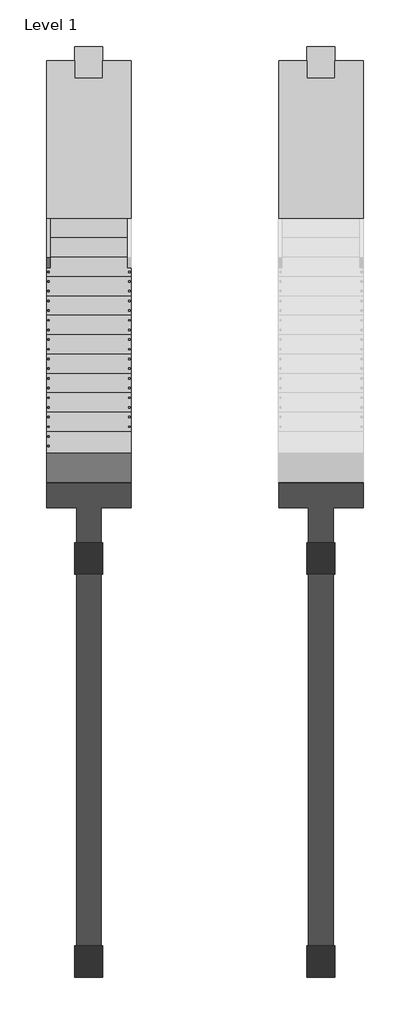
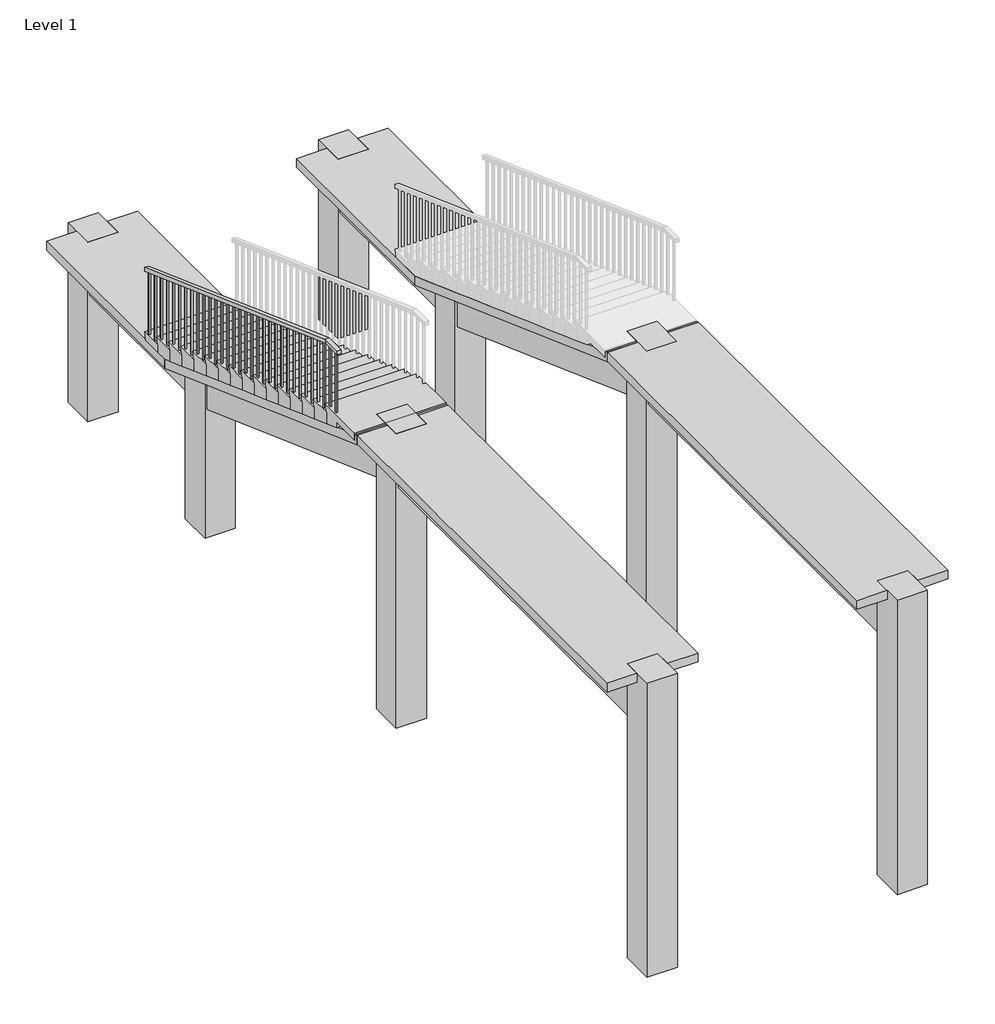
# One storey, part 1 of 2: 8 columns, 6 beams, 1 railing, 1 stair flight.
"""IFC4 building model written with IfcOpenShell, lengths in millimetres."""

from ifc_helpers import new_model, si_unit, frame, origin, place, context, project, spatial, polyline, outline, extrude, faceted_brep, element, save

model = new_model("IFC4")

# Units and contexts
model_context = context("Model", 3, world=origin())
ifc_project = project(units=[si_unit("LENGTHUNIT", "METRE", prefix="MILLI")], contexts=[model_context])

# Site, building, storey
site = spatial("IfcSite", under=ifc_project)
building = spatial("IfcBuilding", under=site)
storey = spatial("IfcBuildingStorey", under=building, Name="Level 1", Elevation=0.0)

# Beams
placement = place(None, origin())
element("IfcBeam", 1, ObjectType="Concrete-TRectangular Beam : b = 1200 x bw = 350 x tw = 120 x h = 750mm", at=placement, inside=storey, context=model_context, shape_type="Brep", body=[
    faceted_brep([(-3907.916217, 8978.9884038, 0.0), (-3907.916217, 6278.9884038, 0.0), (-3507.916217, 6278.9884038, 0.0), (-3507.916217, 6503.9884038, 0.0), (-3107.916217, 6503.9884038, 0.0), (-3107.916217, 6278.9884038, 0.0), (-2707.916217, 6278.9884038, 0.0), (-2707.916217, 8978.9884038, 0.0), (-3107.916217, 8978.9884038, 0.0), (-3107.916217, 8728.9884038, 0.0), (-3507.916217, 8728.9884038, 0.0), (-3507.916217, 8978.9884038, 0.0), (-2707.916217, 6278.9884038, -120.0), (-2707.916217, 8978.9884038, -120.0), (-3107.916217, 6278.9884038, -120.0), (-3107.916217, 6503.9884038, -120.0), (-3132.916217, 6503.9884038, -120.0), (-3132.916217, 8728.9884038, -120.0), (-3107.916217, 8728.9884038, -120.0), (-3107.916217, 8978.9884038, -120.0), (-3132.916217, 8728.9884038, -750.0), (-3132.916217, 6503.9884038, -750.0), (-3482.916217, 8728.9884038, -750.0), (-3482.916217, 6503.9884038, -750.0), (-3482.916217, 8728.9884038, -120.0), (-3482.916217, 6503.9884038, -120.0), (-3907.916217, 6278.9884038, -120.0), (-3907.916217, 8978.9884038, -120.0), (-3507.916217, 8978.9884038, -120.0), (-3507.916217, 8728.9884038, -120.0), (-3507.916217, 6503.9884038, -120.0), (-3507.916217, 6278.9884038, -120.0)], [[[0, 1, 2, 3, 4, 5, 6, 7, 8, 9, 10, 11]], [[7, 6, 12, 13]], [[13, 12, 14, 15, 16, 17, 18, 19]], [[20, 17, 16, 21]], [[22, 20, 21, 23]], [[24, 22, 23, 25]], [[26, 27, 28, 29, 24, 25, 30, 31]], [[1, 0, 27, 26]], [[10, 29, 28, 11]], [[29, 10, 9, 18, 17, 20, 22, 24]], [[18, 9, 8, 19]], [[12, 6, 5, 14]], [[15, 4, 3, 30, 25, 23, 21, 16]], [[30, 3, 2, 31]], [[4, 15, 14, 5]], [[1, 26, 31, 2]], [[7, 13, 19, 8]], [[27, 0, 11, 28]]]),
])
element("IfcBeam", 2, ObjectType="Concrete-TRectangular Beam : b = 1200 x bw = 350 x tw = 120 x h = 750mm", at=placement, inside=storey, context=model_context, shape_type="Brep", body=[
    faceted_brep([(-3907.916217, 1885.136319, 1600.0), (-3907.916217, -3814.863681, 1600.0), (-3507.916217, -3814.863681, 1600.0), (-3507.916217, -3589.863681, 1600.0), (-3107.916217, -3589.863681, 1600.0), (-3107.916217, -3814.863681, 1600.0), (-2707.916217, -3814.863681, 1600.0), (-2707.916217, 1885.136319, 1600.0), (-3107.916217, 1885.136319, 1600.0), (-3107.916217, 1685.8738053, 1600.0), (-3507.916217, 1685.8738053, 1600.0), (-3507.916217, 1885.136319, 1600.0), (-2707.916217, -3814.863681, 1480.0), (-2707.916217, 1885.136319, 1480.0), (-3107.916217, -3814.863681, 1480.0), (-3107.916217, -3589.863681, 1480.0), (-3132.916217, -3589.863681, 1480.0), (-3132.916217, 1685.8738053, 1480.0), (-3107.916217, 1685.8738053, 1480.0), (-3107.916217, 1885.136319, 1480.0), (-3132.916217, 1685.8738053, 850.0), (-3132.916217, -3589.863681, 850.0), (-3482.916217, 1685.8738053, 850.0), (-3482.916217, -3589.863681, 850.0), (-3482.916217, 1685.8738053, 1480.0), (-3482.916217, -3589.863681, 1480.0), (-3907.916217, -3814.863681, 1480.0), (-3907.916217, 1885.136319, 1480.0), (-3507.916217, 1885.136319, 1480.0), (-3507.916217, 1685.8738053, 1480.0), (-3507.916217, -3589.863681, 1480.0), (-3507.916217, -3814.863681, 1480.0)], [[[0, 1, 2, 3, 4, 5, 6, 7, 8, 9, 10, 11]], [[7, 6, 12, 13]], [[13, 12, 14, 15, 16, 17, 18, 19]], [[20, 17, 16, 21]], [[22, 20, 21, 23]], [[24, 22, 23, 25]], [[26, 27, 28, 29, 24, 25, 30, 31]], [[1, 0, 27, 26]], [[10, 29, 28, 11]], [[29, 10, 9, 18, 17, 20, 22, 24]], [[18, 9, 8, 19]], [[15, 4, 3, 30, 25, 23, 21, 16]], [[30, 3, 2, 31]], [[4, 15, 14, 5]], [[12, 6, 5, 14]], [[1, 26, 31, 2]], [[7, 13, 19, 8]], [[27, 0, 11, 28]]]),
])
element("IfcBeam", 3, ObjectType="Concrete-TRectangular Beam : b = 1200 x bw = 350 x tw = 120 x h = 750mm", at=placement, inside=storey, context=model_context, shape_type="Brep", body=[
    faceted_brep([(-3907.916217, 6278.9884038, 0.0), (-3907.916217, 1885.136319, 1600.0), (-3507.916217, 1885.136319, 1600.0), (-3507.916217, 2135.8738053, 1508.6951562), (-3107.916217, 2135.8738053, 1508.6951562), (-3107.916217, 1885.136319, 1600.0), (-2707.916217, 1885.136319, 1600.0), (-2707.916217, 6278.9884038, 0.0), (-3107.916217, 6278.9884038, 0.0), (-3507.916217, 6278.9884038, 0.0), (-2707.916217, 1885.136319, 1480.0), (-2707.916217, 1885.136319, 1472.2914861), (-2707.916217, 6278.9884038, -127.7085139), (-2707.916217, 6278.9884038, -120.0), (-3107.916217, 1885.136319, 1472.2914861), (-3107.916217, 2135.8738053, 1380.9866424), (-3132.916217, 2135.8738053, 1380.9866424), (-3132.916217, 6053.9884038, -45.7758514), (-3107.916217, 6053.9884038, -45.7758514), (-3107.916217, 6278.9884038, -127.7085139), (-3132.916217, 2135.8738053, 710.5169446), (-3132.916217, 6053.9884038, -716.2455492), (-3482.916217, 2135.8738053, 710.5169446), (-3482.916217, 6053.9884038, -716.2455492), (-3482.916217, 2135.8738053, 1380.9866424), (-3482.916217, 6053.9884038, -45.7758514), (-3907.916217, 1885.136319, 1472.2914861), (-3907.916217, 6278.9884038, -127.7085139), (-3507.916217, 6278.9884038, -127.7085139), (-3507.916217, 6053.9884038, -45.7758514), (-3507.916217, 2135.8738053, 1380.9866424), (-3507.916217, 1885.136319, 1472.2914861), (-3907.916217, 6278.9884038, -120.0), (-3907.916217, 1885.136319, 1480.0), (-3507.916217, 1885.136319, 1480.0), (-3107.916217, 1885.136319, 1480.0), (-3107.916217, 6053.9884038, 0.0), (-3507.916217, 6053.9884038, 0.0), (-3507.916217, 6278.9884038, -120.0), (-3107.916217, 6278.9884038, -120.0)], [[[0, 1, 2, 3, 4, 5, 6, 7, 8, 9]], [[7, 6, 10, 11, 12, 13]], [[12, 11, 14, 15, 16, 17, 18, 19]], [[16, 20, 21, 17]], [[20, 22, 23, 21]], [[22, 24, 25, 23]], [[26, 27, 28, 29, 25, 24, 30, 31]], [[1, 0, 32, 27, 26, 33]], [[15, 4, 3, 30, 24, 22, 20, 16]], [[30, 3, 2, 34, 31]], [[4, 15, 14, 35, 5]], [[36, 37, 9, 8]], [[9, 37, 29, 28, 38]], [[37, 36, 18, 17, 21, 23, 25, 29]], [[36, 8, 39, 19, 18]], [[11, 10, 6, 5, 35, 14]], [[7, 13, 12, 19, 39, 8]], [[1, 33, 26, 31, 34, 2]], [[27, 32, 0, 9, 38, 28]]]),
])
element("IfcBeam", 4, ObjectType="Concrete-TRectangular Beam : b = 1200 x bw = 350 x tw = 120 x h = 750mm", at=placement, inside=storey, context=model_context, shape_type="Brep", body=[
    faceted_brep([(-7207.916217, 8978.9884038, 0.0), (-7207.916217, 6278.9884038, 0.0), (-6807.916217, 6278.9884038, 0.0), (-6807.916217, 6503.9884038, 0.0), (-6407.916217, 6503.9884038, 0.0), (-6407.916217, 6278.9884038, 0.0), (-6007.916217, 6278.9884038, 0.0), (-6007.916217, 8978.9884038, 0.0), (-6407.916217, 8978.9884038, 0.0), (-6407.916217, 8728.9884038, 0.0), (-6807.916217, 8728.9884038, 0.0), (-6807.916217, 8978.9884038, 0.0), (-6007.916217, 6278.9884038, -120.0), (-6007.916217, 8978.9884038, -120.0), (-6407.916217, 6278.9884038, -120.0), (-6407.916217, 6503.9884038, -120.0), (-6432.916217, 6503.9884038, -120.0), (-6432.916217, 8728.9884038, -120.0), (-6407.916217, 8728.9884038, -120.0), (-6407.916217, 8978.9884038, -120.0), (-6432.916217, 8728.9884038, -750.0), (-6432.916217, 6503.9884038, -750.0), (-6782.916217, 8728.9884038, -750.0), (-6782.916217, 6503.9884038, -750.0), (-6782.916217, 8728.9884038, -120.0), (-6782.916217, 6503.9884038, -120.0), (-7207.916217, 6278.9884038, -120.0), (-7207.916217, 8978.9884038, -120.0), (-6807.916217, 8978.9884038, -120.0), (-6807.916217, 8728.9884038, -120.0), (-6807.916217, 6503.9884038, -120.0), (-6807.916217, 6278.9884038, -120.0)], [[[0, 1, 2, 3, 4, 5, 6, 7, 8, 9, 10, 11]], [[7, 6, 12, 13]], [[13, 12, 14, 15, 16, 17, 18, 19]], [[20, 17, 16, 21]], [[22, 20, 21, 23]], [[24, 22, 23, 25]], [[26, 27, 28, 29, 24, 25, 30, 31]], [[1, 0, 27, 26]], [[10, 29, 28, 11]], [[29, 10, 9, 18, 17, 20, 22, 24]], [[18, 9, 8, 19]], [[12, 6, 5, 14]], [[15, 4, 3, 30, 25, 23, 21, 16]], [[30, 3, 2, 31]], [[4, 15, 14, 5]], [[1, 26, 31, 2]], [[7, 13, 19, 8]], [[27, 0, 11, 28]]]),
])
element("IfcBeam", 5, ObjectType="Concrete-TRectangular Beam : b = 1200 x bw = 350 x tw = 120 x h = 750mm", at=placement, inside=storey, context=model_context, shape_type="Brep", body=[
    faceted_brep([(-7207.916217, 1885.136319, 1600.0), (-7207.916217, -3814.863681, 1600.0), (-6807.916217, -3814.863681, 1600.0), (-6807.916217, -3589.863681, 1600.0), (-6407.916217, -3589.863681, 1600.0), (-6407.916217, -3814.863681, 1600.0), (-6007.916217, -3814.863681, 1600.0), (-6007.916217, 1885.136319, 1600.0), (-6407.916217, 1885.136319, 1600.0), (-6407.916217, 1685.8738053, 1600.0), (-6807.916217, 1685.8738053, 1600.0), (-6807.916217, 1885.136319, 1600.0), (-6007.916217, -3814.863681, 1480.0), (-6007.916217, 1885.136319, 1480.0), (-6407.916217, -3814.863681, 1480.0), (-6407.916217, -3589.863681, 1480.0), (-6432.916217, -3589.863681, 1480.0), (-6432.916217, 1685.8738053, 1480.0), (-6407.916217, 1685.8738053, 1480.0), (-6407.916217, 1885.136319, 1480.0), (-6432.916217, 1685.8738053, 850.0), (-6432.916217, -3589.863681, 850.0), (-6782.916217, 1685.8738053, 850.0), (-6782.916217, -3589.863681, 850.0), (-6782.916217, 1685.8738053, 1480.0), (-6782.916217, -3589.863681, 1480.0), (-7207.916217, -3814.863681, 1480.0), (-7207.916217, 1885.136319, 1480.0), (-6807.916217, 1885.136319, 1480.0), (-6807.916217, 1685.8738053, 1480.0), (-6807.916217, -3589.863681, 1480.0), (-6807.916217, -3814.863681, 1480.0)], [[[0, 1, 2, 3, 4, 5, 6, 7, 8, 9, 10, 11]], [[7, 6, 12, 13]], [[13, 12, 14, 15, 16, 17, 18, 19]], [[20, 17, 16, 21]], [[22, 20, 21, 23]], [[24, 22, 23, 25]], [[26, 27, 28, 29, 24, 25, 30, 31]], [[1, 0, 27, 26]], [[10, 29, 28, 11]], [[29, 10, 9, 18, 17, 20, 22, 24]], [[18, 9, 8, 19]], [[15, 4, 3, 30, 25, 23, 21, 16]], [[30, 3, 2, 31]], [[4, 15, 14, 5]], [[12, 6, 5, 14]], [[1, 26, 31, 2]], [[7, 13, 19, 8]], [[27, 0, 11, 28]]]),
])
element("IfcBeam", 6, ObjectType="Concrete-TRectangular Beam : b = 1200 x bw = 350 x tw = 120 x h = 750mm", at=placement, inside=storey, context=model_context, shape_type="Brep", body=[
    faceted_brep([(-7207.916217, 6278.9884038, 0.0), (-7207.916217, 1885.136319, 1600.0), (-6807.916217, 1885.136319, 1600.0), (-6807.916217, 2135.8738053, 1508.6951562), (-6407.916217, 2135.8738053, 1508.6951562), (-6407.916217, 1885.136319, 1600.0), (-6007.916217, 1885.136319, 1600.0), (-6007.916217, 6278.9884038, 0.0), (-6407.916217, 6278.9884038, 0.0), (-6807.916217, 6278.9884038, 0.0), (-6007.916217, 1885.136319, 1480.0), (-6007.916217, 1885.136319, 1472.2914861), (-6007.916217, 6278.9884038, -127.7085139), (-6007.916217, 6278.9884038, -120.0), (-6407.916217, 1885.136319, 1472.2914861), (-6407.916217, 2135.8738053, 1380.9866424), (-6432.916217, 2135.8738053, 1380.9866424), (-6432.916217, 6053.9884038, -45.7758514), (-6407.916217, 6053.9884038, -45.7758514), (-6407.916217, 6278.9884038, -127.7085139), (-6432.916217, 2135.8738053, 710.5169446), (-6432.916217, 6053.9884038, -716.2455492), (-6782.916217, 2135.8738053, 710.5169446), (-6782.916217, 6053.9884038, -716.2455492), (-6782.916217, 2135.8738053, 1380.9866424), (-6782.916217, 6053.9884038, -45.7758514), (-7207.916217, 1885.136319, 1472.2914861), (-7207.916217, 6278.9884038, -127.7085139), (-6807.916217, 6278.9884038, -127.7085139), (-6807.916217, 6053.9884038, -45.7758514), (-6807.916217, 2135.8738053, 1380.9866424), (-6807.916217, 1885.136319, 1472.2914861), (-7207.916217, 6278.9884038, -120.0), (-7207.916217, 1885.136319, 1480.0), (-6807.916217, 1885.136319, 1480.0), (-6407.916217, 1885.136319, 1480.0), (-6407.916217, 6053.9884038, 0.0), (-6807.916217, 6053.9884038, 0.0), (-6807.916217, 6278.9884038, -120.0), (-6407.916217, 6278.9884038, -120.0)], [[[0, 1, 2, 3, 4, 5, 6, 7, 8, 9]], [[7, 6, 10, 11, 12, 13]], [[12, 11, 14, 15, 16, 17, 18, 19]], [[16, 20, 21, 17]], [[20, 22, 23, 21]], [[22, 24, 25, 23]], [[26, 27, 28, 29, 25, 24, 30, 31]], [[1, 0, 32, 27, 26, 33]], [[15, 4, 3, 30, 24, 22, 20, 16]], [[30, 3, 2, 34, 31]], [[4, 15, 14, 35, 5]], [[36, 37, 9, 8]], [[9, 37, 29, 28, 38]], [[37, 36, 18, 17, 21, 23, 25, 29]], [[36, 8, 39, 19, 18]], [[11, 10, 6, 5, 35, 14]], [[7, 13, 12, 19, 39, 8]], [[1, 33, 26, 31, 34, 2]], [[27, 32, 0, 9, 38, 28]]]),
])

# Columns
element("IfcColumn", 7, ObjectType="Concrete-Rectangular-Column : 400 x 450mm 2", at=placement, inside=storey, context=model_context, shape_type="SweptSolid", body=[
    extrude(outline(polyline([(-3107.916217, 2135.8738053), (-3107.916217, 1685.8738053), (-3507.916217, 1685.8738053), (-3507.916217, 2135.8738053), (-3107.916217, 2135.8738053)])), frame((0.0, 0.0, -2500.0), z_axis=(0.0, 0.0, 1.0), x_axis=(1.0, 0.0, 0.0)), (0.0, 0.0, 1.0), 4100.0),
])
element("IfcColumn", 8, ObjectType="Concrete-Rectangular-Column : 400 x 450mm 2", at=placement, inside=storey, context=model_context, shape_type="SweptSolid", body=[
    extrude(outline(polyline([(-3107.916217, 6503.9884038), (-3107.916217, 6053.9884038), (-3507.916217, 6053.9884038), (-3507.916217, 6503.9884038), (-3107.916217, 6503.9884038)])), frame((0.0, 0.0, -2500.0), z_axis=(0.0, 0.0, 1.0), x_axis=(1.0, 0.0, 0.0)), (0.0, 0.0, 1.0), 2500.0),
])
element("IfcColumn", 9, ObjectType="Concrete-Rectangular-Column : 400 x 450mm 2", at=placement, inside=storey, context=model_context, shape_type="SweptSolid", body=[
    extrude(outline(polyline([(-3107.916217, 9178.9884038), (-3107.916217, 8728.9884038), (-3507.916217, 8728.9884038), (-3507.916217, 9178.9884038), (-3107.916217, 9178.9884038)])), frame((0.0, 0.0, -2500.0), z_axis=(0.0, 0.0, 1.0), x_axis=(1.0, 0.0, 0.0)), (0.0, 0.0, 1.0), 2500.0),
])
element("IfcColumn", 10, ObjectType="Concrete-Rectangular-Column : 400 x 450mm 2", at=placement, inside=storey, context=model_context, shape_type="SweptSolid", body=[
    extrude(outline(polyline([(-3107.916217, -3589.863681), (-3107.916217, -4039.863681), (-3507.916217, -4039.863681), (-3507.916217, -3589.863681), (-3107.916217, -3589.863681)])), frame((0.0, 0.0, -2500.0), z_axis=(0.0, 0.0, 1.0), x_axis=(1.0, 0.0, 0.0)), (0.0, 0.0, 1.0), 4100.0),
])
element("IfcColumn", 11, ObjectType="Concrete-Rectangular-Column : 400 x 450mm 2", at=placement, inside=storey, context=model_context, shape_type="SweptSolid", body=[
    extrude(outline(polyline([(-6407.916217, 2135.8738053), (-6407.916217, 1685.8738053), (-6807.916217, 1685.8738053), (-6807.916217, 2135.8738053), (-6407.916217, 2135.8738053)])), frame((0.0, 0.0, -2500.0), z_axis=(0.0, 0.0, 1.0), x_axis=(1.0, 0.0, 0.0)), (0.0, 0.0, 1.0), 4100.0),
])
element("IfcColumn", 12, ObjectType="Concrete-Rectangular-Column : 400 x 450mm 2", at=placement, inside=storey, context=model_context, shape_type="SweptSolid", body=[
    extrude(outline(polyline([(-6407.916217, 6503.9884038), (-6407.916217, 6053.9884038), (-6807.916217, 6053.9884038), (-6807.916217, 6503.9884038), (-6407.916217, 6503.9884038)])), frame((0.0, 0.0, -2500.0), z_axis=(0.0, 0.0, 1.0), x_axis=(1.0, 0.0, 0.0)), (0.0, 0.0, 1.0), 2500.0),
])
element("IfcColumn", 13, ObjectType="Concrete-Rectangular-Column : 400 x 450mm 2", at=placement, inside=storey, context=model_context, shape_type="SweptSolid", body=[
    extrude(outline(polyline([(-6407.916217, 9178.9884038), (-6407.916217, 8728.9884038), (-6807.916217, 8728.9884038), (-6807.916217, 9178.9884038), (-6407.916217, 9178.9884038)])), frame((0.0, 0.0, -2500.0), z_axis=(0.0, 0.0, 1.0), x_axis=(1.0, 0.0, 0.0)), (0.0, 0.0, 1.0), 2500.0),
])
element("IfcColumn", 14, ObjectType="Concrete-Rectangular-Column : 400 x 450mm 2", at=placement, inside=storey, context=model_context, shape_type="SweptSolid", body=[
    extrude(outline(polyline([(-6407.916217, -3589.863681), (-6407.916217, -4039.863681), (-6807.916217, -4039.863681), (-6807.916217, -3589.863681), (-6407.916217, -3589.863681)])), frame((0.0, 0.0, -2500.0), z_axis=(0.0, 0.0, 1.0), x_axis=(1.0, 0.0, 0.0)), (0.0, 0.0, 1.0), 4100.0),
])

# Railing
element("IfcRailing", 15, ObjectType="900mm", at=placement, inside=storey, context=model_context, shape_type="SolidModel", body=[
    faceted_brep([(-7159.0267942, 6735.8738053, 1000.0), (-7159.0267942, 6735.8738053, 946.7968186), (-7209.0267942, 6735.8738053, 946.7968186), (-7209.0267942, 6735.8738053, 1000.0), (-7159.0267942, 2610.8738053, 2500.0), (-7159.0267942, 2602.0650564, 2450.0), (-7209.0267942, 2602.0650564, 2450.0), (-7209.0267942, 2610.8738053, 2500.0), (-7159.0267942, 2335.8738053, 2500.0), (-7209.0267942, 2335.8738053, 2500.0), (-7209.0267942, 2335.8738053, 2450.0), (-7159.0267942, 2335.8738053, 2450.0)], [[[0, 1, 2, 3]], [[1, 0, 4, 5]], [[2, 1, 5, 6]], [[3, 2, 6, 7]], [[0, 3, 7, 4]], [[8, 9, 10, 11]], [[5, 4, 8, 11]], [[6, 5, 11, 10]], [[7, 6, 10, 9]], [[4, 7, 9, 8]]]),
    extrude(outline(polyline([(-7194.0267942, 2414.6238053), (-7174.0267942, 2414.6238053), (-7174.0267942, 2394.6238053), (-7194.0267942, 2394.6238053), (-7194.0267942, 2414.6238053)])), frame((0.0, 0.0, 1600.0), z_axis=(0.0, 0.0, 1.0), x_axis=(1.0, 0.0, 0.0)), (0.0, 0.0, 1.0), 850.0),
    extrude(outline(polyline([(-7194.0267942, 2552.1238053), (-7174.0267942, 2552.1238053), (-7174.0267942, 2532.1238053), (-7194.0267942, 2532.1238053), (-7194.0267942, 2552.1238053)])), frame((0.0, 0.0, 1600.0), z_axis=(0.0, 0.0, 1.0), x_axis=(1.0, 0.0, 0.0)), (0.0, 0.0, 1.0), 850.0),
    extrude(outline(polyline([(2689.6238053, 2418.160455), (2689.6238053, 1500.0), (2669.6238053, 1500.0), (2669.6238053, 2425.4331822), (2689.6238053, 2418.160455)])), frame((-7194.0267942, 0.0, 0.0), z_axis=(1.0, 0.0, 0.0), x_axis=(0.0, 1.0, 0.0)), (0.0, 0.0, 1.0), 20.0),
    extrude(outline(polyline([(2827.1238053, 2368.160455), (2827.1238053, 1500.0), (2807.1238053, 1500.0), (2807.1238053, 2375.4331822), (2827.1238053, 2368.160455)])), frame((-7194.0267942, 0.0, 0.0), z_axis=(1.0, 0.0, 0.0), x_axis=(0.0, 1.0, 0.0)), (0.0, 0.0, 1.0), 20.0),
    extrude(outline(polyline([(2964.6238053, 2318.160455), (2964.6238053, 1400.0), (2944.6238053, 1400.0), (2944.6238053, 2325.4331822), (2964.6238053, 2318.160455)])), frame((-7194.0267942, 0.0, 0.0), z_axis=(1.0, 0.0, 0.0), x_axis=(0.0, 1.0, 0.0)), (0.0, 0.0, 1.0), 20.0),
    extrude(outline(polyline([(3102.1238053, 2268.160455), (3102.1238053, 1400.0), (3082.1238053, 1400.0), (3082.1238053, 2275.4331822), (3102.1238053, 2268.160455)])), frame((-7194.0267942, 0.0, 0.0), z_axis=(1.0, 0.0, 0.0), x_axis=(0.0, 1.0, 0.0)), (0.0, 0.0, 1.0), 20.0),
    extrude(outline(polyline([(3239.6238053, 2218.160455), (3239.6238053, 1300.0), (3219.6238053, 1300.0), (3219.6238053, 2225.4331822), (3239.6238053, 2218.160455)])), frame((-7194.0267942, 0.0, 0.0), z_axis=(1.0, 0.0, 0.0), x_axis=(0.0, 1.0, 0.0)), (0.0, 0.0, 1.0), 20.0),
    extrude(outline(polyline([(3377.1238053, 2168.160455), (3377.1238053, 1300.0), (3357.1238053, 1300.0), (3357.1238053, 2175.4331822), (3377.1238053, 2168.160455)])), frame((-7194.0267942, 0.0, 0.0), z_axis=(1.0, 0.0, 0.0), x_axis=(0.0, 1.0, 0.0)), (0.0, 0.0, 1.0), 20.0),
    extrude(outline(polyline([(3514.6238053, 2118.160455), (3514.6238053, 1200.0), (3494.6238053, 1200.0), (3494.6238053, 2125.4331822), (3514.6238053, 2118.160455)])), frame((-7194.0267942, 0.0, 0.0), z_axis=(1.0, 0.0, 0.0), x_axis=(0.0, 1.0, 0.0)), (0.0, 0.0, 1.0), 20.0),
    extrude(outline(polyline([(3652.1238053, 2068.160455), (3652.1238053, 1200.0), (3632.1238053, 1200.0), (3632.1238053, 2075.4331822), (3652.1238053, 2068.160455)])), frame((-7194.0267942, 0.0, 0.0), z_axis=(1.0, 0.0, 0.0), x_axis=(0.0, 1.0, 0.0)), (0.0, 0.0, 1.0), 20.0),
    extrude(outline(polyline([(3789.6238053, 2018.160455), (3789.6238053, 1100.0), (3769.6238053, 1100.0), (3769.6238053, 2025.4331822), (3789.6238053, 2018.160455)])), frame((-7194.0267942, 0.0, 0.0), z_axis=(1.0, 0.0, 0.0), x_axis=(0.0, 1.0, 0.0)), (0.0, 0.0, 1.0), 20.0),
    extrude(outline(polyline([(3927.1238053, 1968.160455), (3927.1238053, 1100.0), (3907.1238053, 1100.0), (3907.1238053, 1975.4331822), (3927.1238053, 1968.160455)])), frame((-7194.0267942, 0.0, 0.0), z_axis=(1.0, 0.0, 0.0), x_axis=(0.0, 1.0, 0.0)), (0.0, 0.0, 1.0), 20.0),
    extrude(outline(polyline([(4064.6238053, 1918.160455), (4064.6238053, 1000.0), (4044.6238053, 1000.0), (4044.6238053, 1925.4331822), (4064.6238053, 1918.160455)])), frame((-7194.0267942, 0.0, 0.0), z_axis=(1.0, 0.0, 0.0), x_axis=(0.0, 1.0, 0.0)), (0.0, 0.0, 1.0), 20.0),
    extrude(outline(polyline([(4202.1238053, 1868.160455), (4202.1238053, 1000.0), (4182.1238053, 1000.0), (4182.1238053, 1875.4331822), (4202.1238053, 1868.160455)])), frame((-7194.0267942, 0.0, 0.0), z_axis=(1.0, 0.0, 0.0), x_axis=(0.0, 1.0, 0.0)), (0.0, 0.0, 1.0), 20.0),
    extrude(outline(polyline([(4339.6238053, 1818.160455), (4339.6238053, 900.0), (4319.6238053, 900.0), (4319.6238053, 1825.4331822), (4339.6238053, 1818.160455)])), frame((-7194.0267942, 0.0, 0.0), z_axis=(1.0, 0.0, 0.0), x_axis=(0.0, 1.0, 0.0)), (0.0, 0.0, 1.0), 20.0),
    extrude(outline(polyline([(4477.1238053, 1768.160455), (4477.1238053, 900.0), (4457.1238053, 900.0), (4457.1238053, 1775.4331822), (4477.1238053, 1768.160455)])), frame((-7194.0267942, 0.0, 0.0), z_axis=(1.0, 0.0, 0.0), x_axis=(0.0, 1.0, 0.0)), (0.0, 0.0, 1.0), 20.0),
    extrude(outline(polyline([(4614.6238053, 1718.160455), (4614.6238053, 800.0), (4594.6238053, 800.0), (4594.6238053, 1725.4331822), (4614.6238053, 1718.160455)])), frame((-7194.0267942, 0.0, 0.0), z_axis=(1.0, 0.0, 0.0), x_axis=(0.0, 1.0, 0.0)), (0.0, 0.0, 1.0), 20.0),
    extrude(outline(polyline([(4752.1238053, 1668.160455), (4752.1238053, 800.0), (4732.1238053, 800.0), (4732.1238053, 1675.4331822), (4752.1238053, 1668.160455)])), frame((-7194.0267942, 0.0, 0.0), z_axis=(1.0, 0.0, 0.0), x_axis=(0.0, 1.0, 0.0)), (0.0, 0.0, 1.0), 20.0),
    extrude(outline(polyline([(4889.6238053, 1618.160455), (4889.6238053, 700.0), (4869.6238053, 700.0), (4869.6238053, 1625.4331822), (4889.6238053, 1618.160455)])), frame((-7194.0267942, 0.0, 0.0), z_axis=(1.0, 0.0, 0.0), x_axis=(0.0, 1.0, 0.0)), (0.0, 0.0, 1.0), 20.0),
    extrude(outline(polyline([(5027.1238053, 1568.160455), (5027.1238053, 700.0), (5007.1238053, 700.0), (5007.1238053, 1575.4331822), (5027.1238053, 1568.160455)])), frame((-7194.0267942, 0.0, 0.0), z_axis=(1.0, 0.0, 0.0), x_axis=(0.0, 1.0, 0.0)), (0.0, 0.0, 1.0), 20.0),
    extrude(outline(polyline([(5164.6238053, 1518.160455), (5164.6238053, 600.0), (5144.6238053, 600.0), (5144.6238053, 1525.4331822), (5164.6238053, 1518.160455)])), frame((-7194.0267942, 0.0, 0.0), z_axis=(1.0, 0.0, 0.0), x_axis=(0.0, 1.0, 0.0)), (0.0, 0.0, 1.0), 20.0),
    extrude(outline(polyline([(5302.1238053, 1468.160455), (5302.1238053, 600.0), (5282.1238053, 600.0), (5282.1238053, 1475.4331822), (5302.1238053, 1468.160455)])), frame((-7194.0267942, 0.0, 0.0), z_axis=(1.0, 0.0, 0.0), x_axis=(0.0, 1.0, 0.0)), (0.0, 0.0, 1.0), 20.0),
    extrude(outline(polyline([(5439.6238053, 1418.160455), (5439.6238053, 500.0), (5419.6238053, 500.0), (5419.6238053, 1425.4331822), (5439.6238053, 1418.160455)])), frame((-7194.0267942, 0.0, 0.0), z_axis=(1.0, 0.0, 0.0), x_axis=(0.0, 1.0, 0.0)), (0.0, 0.0, 1.0), 20.0),
    extrude(outline(polyline([(5577.1238053, 1368.160455), (5577.1238053, 500.0), (5557.1238053, 500.0), (5557.1238053, 1375.4331822), (5577.1238053, 1368.160455)])), frame((-7194.0267942, 0.0, 0.0), z_axis=(1.0, 0.0, 0.0), x_axis=(0.0, 1.0, 0.0)), (0.0, 0.0, 1.0), 20.0),
    extrude(outline(polyline([(5714.6238053, 1318.160455), (5714.6238053, 400.0), (5694.6238053, 400.0), (5694.6238053, 1325.4331822), (5714.6238053, 1318.160455)])), frame((-7194.0267942, 0.0, 0.0), z_axis=(1.0, 0.0, 0.0), x_axis=(0.0, 1.0, 0.0)), (0.0, 0.0, 1.0), 20.0),
    extrude(outline(polyline([(5852.1238053, 1268.160455), (5852.1238053, 400.0), (5832.1238053, 400.0), (5832.1238053, 1275.4331822), (5852.1238053, 1268.160455)])), frame((-7194.0267942, 0.0, 0.0), z_axis=(1.0, 0.0, 0.0), x_axis=(0.0, 1.0, 0.0)), (0.0, 0.0, 1.0), 20.0),
    extrude(outline(polyline([(5989.6238053, 1218.160455), (5989.6238053, 300.0), (5969.6238053, 300.0), (5969.6238053, 1225.4331822), (5989.6238053, 1218.160455)])), frame((-7194.0267942, 0.0, 0.0), z_axis=(1.0, 0.0, 0.0), x_axis=(0.0, 1.0, 0.0)), (0.0, 0.0, 1.0), 20.0),
    extrude(outline(polyline([(6127.1238053, 1168.160455), (6127.1238053, 300.0), (6107.1238053, 300.0), (6107.1238053, 1175.4331822), (6127.1238053, 1168.160455)])), frame((-7194.0267942, 0.0, 0.0), z_axis=(1.0, 0.0, 0.0), x_axis=(0.0, 1.0, 0.0)), (0.0, 0.0, 1.0), 20.0),
    extrude(outline(polyline([(6264.6238053, 1118.160455), (6264.6238053, 200.0), (6244.6238053, 200.0), (6244.6238053, 1125.4331822), (6264.6238053, 1118.160455)])), frame((-7194.0267942, 0.0, 0.0), z_axis=(1.0, 0.0, 0.0), x_axis=(0.0, 1.0, 0.0)), (0.0, 0.0, 1.0), 20.0),
    extrude(outline(polyline([(6402.1238053, 1068.160455), (6402.1238053, 200.0), (6382.1238053, 200.0), (6382.1238053, 1075.4331822), (6402.1238053, 1068.160455)])), frame((-7194.0267942, 0.0, 0.0), z_axis=(1.0, 0.0, 0.0), x_axis=(0.0, 1.0, 0.0)), (0.0, 0.0, 1.0), 20.0),
    extrude(outline(polyline([(6539.6238053, 1018.160455), (6539.6238053, 100.0), (6519.6238053, 100.0), (6519.6238053, 1025.4331822), (6539.6238053, 1018.160455)])), frame((-7194.0267942, 0.0, 0.0), z_axis=(1.0, 0.0, 0.0), x_axis=(0.0, 1.0, 0.0)), (0.0, 0.0, 1.0), 20.0),
    extrude(outline(polyline([(6677.1238053, 968.160455), (6677.1238053, 100.0), (6657.1238053, 100.0), (6657.1238053, 975.4331822), (6677.1238053, 968.160455)])), frame((-7194.0267942, 0.0, 0.0), z_axis=(1.0, 0.0, 0.0), x_axis=(0.0, 1.0, 0.0)), (0.0, 0.0, 1.0), 20.0),
])

# Stair flight
element("IfcStairFlight", 16, ObjectType="25 mm Nosing", at=placement, inside=storey, context=model_context, shape_type="Brep", body=[
    faceted_brep([(-7209.4267942, 6735.8738053, 100.0), (-6006.4056398, 6735.8738053, 100.0), (-6006.4056398, 6710.8738053, 0.0), (-7209.4267942, 6710.8738053, 0.0), (-7209.4267942, 6435.8738053, 100.0), (-6006.4056398, 6435.8738053, 100.0), (-6006.4056398, 6435.8738053, 0.0), (-7209.4267942, 6435.8738053, 0.0), (-6006.4056398, 6460.8738053, 200.0), (-7209.4267942, 6460.8738053, 200.0), (-7209.4267942, 6160.8738053, 200.0), (-6006.4056398, 6160.8738053, 200.0), (-6006.4056398, 6160.8738053, 40.3904558), (-6006.4056398, 6271.9475586, 0.0), (-7209.4267942, 6271.9475586, 0.0), (-7209.4267942, 6160.8738053, 40.3904558), (-6006.4056398, 6185.8738053, 300.0), (-7209.4267942, 6185.8738053, 300.0), (-7209.4267942, 5885.8738053, 300.0), (-6006.4056398, 5885.8738053, 300.0), (-6006.4056398, 5885.8738053, 140.3904558), (-7209.4267942, 5885.8738053, 140.3904558), (-6006.4056398, 5910.8738053, 400.0), (-7209.4267942, 5910.8738053, 400.0), (-7209.4267942, 5610.8738053, 400.0), (-6006.4056398, 5610.8738053, 400.0), (-6006.4056398, 5610.8738053, 240.3904558), (-7209.4267942, 5610.8738053, 240.3904558), (-6006.4056398, 5635.8738053, 500.0), (-7209.4267942, 5635.8738053, 500.0), (-7209.4267942, 5335.8738053, 500.0), (-6006.4056398, 5335.8738053, 500.0), (-6006.4056398, 5335.8738053, 340.3904558), (-7209.4267942, 5335.8738053, 340.3904558), (-6006.4056398, 5360.8738053, 600.0), (-7209.4267942, 5360.8738053, 600.0), (-7209.4267942, 5060.8738053, 600.0), (-6006.4056398, 5060.8738053, 600.0), (-6006.4056398, 5060.8738053, 440.3904558), (-7209.4267942, 5060.8738053, 440.3904558), (-6006.4056398, 5085.8738053, 700.0), (-7209.4267942, 5085.8738053, 700.0), (-7209.4267942, 4785.8738053, 700.0), (-6006.4056398, 4785.8738053, 700.0), (-6006.4056398, 4785.8738053, 540.3904558), (-7209.4267942, 4785.8738053, 540.3904558), (-6006.4056398, 4810.8738053, 800.0), (-7209.4267942, 4810.8738053, 800.0), (-7209.4267942, 4510.8738053, 800.0), (-6006.4056398, 4510.8738053, 800.0), (-6006.4056398, 4510.8738053, 640.3904558), (-7209.4267942, 4510.8738053, 640.3904558), (-6006.4056398, 4535.8738053, 900.0), (-7209.4267942, 4535.8738053, 900.0), (-7209.4267942, 4235.8738053, 900.0), (-6006.4056398, 4235.8738053, 900.0), (-6006.4056398, 4235.8738053, 740.3904558), (-7209.4267942, 4235.8738053, 740.3904558), (-6006.4056398, 4260.8738053, 1000.0), (-7209.4267942, 4260.8738053, 1000.0), (-7209.4267942, 3960.8738053, 1000.0), (-6006.4056398, 3960.8738053, 1000.0), (-6006.4056398, 3960.8738053, 840.3904558), (-7209.4267942, 3960.8738053, 840.3904558), (-6006.4056398, 3985.8738053, 1100.0), (-7209.4267942, 3985.8738053, 1100.0), (-7209.4267942, 3685.8738053, 1100.0), (-6006.4056398, 3685.8738053, 1100.0), (-6006.4056398, 3685.8738053, 940.3904558), (-7209.4267942, 3685.8738053, 940.3904558), (-6006.4056398, 3710.8738053, 1200.0), (-7209.4267942, 3710.8738053, 1200.0), (-7209.4267942, 3410.8738053, 1200.0), (-6006.4056398, 3410.8738053, 1200.0), (-6006.4056398, 3410.8738053, 1040.3904558), (-7209.4267942, 3410.8738053, 1040.3904558), (-6006.4056398, 3435.8738053, 1300.0), (-7209.4267942, 3435.8738053, 1300.0), (-7209.4267942, 3135.8738053, 1300.0), (-6006.4056398, 3135.8738053, 1300.0), (-6006.4056398, 3135.8738053, 1140.3904558), (-7209.4267942, 3135.8738053, 1140.3904558), (-6006.4056398, 3160.8738053, 1400.0), (-7209.4267942, 3160.8738053, 1400.0), (-7209.4267942, 2860.8738053, 1400.0), (-6006.4056398, 2860.8738053, 1400.0), (-6006.4056398, 2860.8738053, 1240.3904558), (-7209.4267942, 2860.8738053, 1240.3904558), (-6006.4056398, 2885.8738053, 1500.0), (-7209.4267942, 2885.8738053, 1500.0), (-7209.4267942, 2585.8738053, 1500.0), (-6006.4056398, 2585.8738053, 1500.0), (-6006.4056398, 2585.8738053, 1340.3904558), (-7209.4267942, 2585.8738053, 1340.3904558), (-6006.4056398, 2610.8738053, 1600.0), (-7209.4267942, 2610.8738053, 1600.0), (-7209.4267942, 1935.8738053, 1600.0), (-6006.4056398, 1935.8738053, 1600.0), (-6006.4056398, 1935.8738053, 1500.0), (-6006.4056398, 2335.8738053, 1500.0), (-6006.4056398, 2335.8738053, 1431.2995467), (-7209.4267942, 2335.8738053, 1431.2995467), (-7209.4267942, 2335.8738053, 1500.0), (-7209.4267942, 1935.8738053, 1500.0)], [[[0, 1, 2, 3]], [[1, 0, 4, 5]], [[1, 5, 6, 2]], [[4, 0, 3, 7]], [[8, 9, 10, 11]], [[6, 5, 8, 11, 12, 13]], [[4, 7, 14, 15, 10, 9]], [[5, 4, 9, 8]], [[16, 17, 18, 19]], [[16, 19, 20, 12, 11]], [[18, 17, 10, 15, 21]], [[11, 10, 17, 16]], [[22, 23, 24, 25]], [[22, 25, 26, 20, 19]], [[24, 23, 18, 21, 27]], [[19, 18, 23, 22]], [[28, 29, 30, 31]], [[28, 31, 32, 26, 25]], [[30, 29, 24, 27, 33]], [[25, 24, 29, 28]], [[34, 35, 36, 37]], [[34, 37, 38, 32, 31]], [[36, 35, 30, 33, 39]], [[31, 30, 35, 34]], [[40, 41, 42, 43]], [[40, 43, 44, 38, 37]], [[42, 41, 36, 39, 45]], [[37, 36, 41, 40]], [[46, 47, 48, 49]], [[46, 49, 50, 44, 43]], [[48, 47, 42, 45, 51]], [[43, 42, 47, 46]], [[52, 53, 54, 55]], [[52, 55, 56, 50, 49]], [[54, 53, 48, 51, 57]], [[49, 48, 53, 52]], [[58, 59, 60, 61]], [[58, 61, 62, 56, 55]], [[60, 59, 54, 57, 63]], [[55, 54, 59, 58]], [[64, 65, 66, 67]], [[64, 67, 68, 62, 61]], [[66, 65, 60, 63, 69]], [[61, 60, 65, 64]], [[70, 71, 72, 73]], [[70, 73, 74, 68, 67]], [[72, 71, 66, 69, 75]], [[67, 66, 71, 70]], [[76, 77, 78, 79]], [[76, 79, 80, 74, 73]], [[78, 77, 72, 75, 81]], [[73, 72, 77, 76]], [[82, 83, 84, 85]], [[82, 85, 86, 80, 79]], [[84, 83, 78, 81, 87]], [[79, 78, 83, 82]], [[88, 89, 90, 91]], [[88, 91, 92, 86, 85]], [[90, 89, 84, 87, 93]], [[85, 84, 89, 88]], [[94, 95, 96, 97]], [[94, 97, 98, 99, 100, 92, 91]], [[96, 95, 90, 93, 101, 102, 103]], [[101, 100, 99, 102]], [[91, 90, 95, 94]], [[2, 6, 13, 14, 7, 3]], [[14, 13, 12, 20, 26, 32, 38, 44, 50, 56, 62, 68, 74, 80, 86, 92, 100, 101, 93, 87, 81, 75, 69, 63, 57, 51, 45, 39, 33, 27, 21, 15]], [[103, 102, 99, 98]], [[103, 98, 97, 96]]]),
])

save(model, "model.ifc")

# Revit data of these elements
# Project information
#   Fecha de emisión de proyecto = "Issue Date"
#   Estado de proyecto = "Project Status"
#   Nombre de cliente = "Owner"
#   Dirección de proyecto = "Enter address here"
#   Nombre de proyecto = "Project Name"
#   Número de proyecto = "Project Number"
# Type "Concrete-TRectangular Beam : b = 1200 x bw = 350 x tw = 120 x h = 750mm"
#   hw = 120 mm
#   bw = 350 mm
#   Length [instance default] = 1524 mm
#   b = 1200 mm
#   h = 750 mm
#   Structural Material [instance default] = Concrete, Cast-in-Place gray
#   Assembly Code = ""
# Type "Concrete-Rectangular-Column : 400 x 450mm 2"
#   b = 400 mm
#   h = 450 mm
#   Structural Material [instance default] = Concrete, Cast-in-Place gray
# Type "900mm"
#   built-in parameter 1008612 = 0.019685 (stored number, unit not read)
#   built-in parameter 1008611 = 0.019685 (stored number, unit not read)
#   built-in parameter 1008609 = 0.902231 (stored number, unit not read)
#   built-in parameter 1008604 = 0.19685 (stored number, unit not read)
#   built-in parameter 1008603 = 0.164042 (stored number, unit not read)
#   Railing Height = 900 mm
#   built-in parameter 1008630 = 2
#   built-in parameter 1008610 = 2
#   built-in parameter 1008608 = 1
#   built-in parameter 1008618 = Baluster - Square : 20mm
# Elements 1, 2, 3, 4, 5, 6 (IfcBeam, "Concrete-TRectangular Beam : b = 1200 x bw = 350 x tw = 120 x h = 750mm")
#   Structural Material = Concrete, Cast-in-Place gray
#   Phase Created = New Construction
#   Materials on its faces: "Concrete, Cast-in-Place gray"
# Elements 7, 8, 9, 10, 11, 12, 13, 14 (IfcColumn, "Concrete-Rectangular-Column : 400 x 450mm 2")
#   Structural Material = Concrete, Cast-in-Place gray
#   Phase Created = New Construction
#   Materials on its faces: "Concrete, Cast-in-Place gray"
# Element 15 (IfcRailing, "900mm")
#   Phase Created = New Construction
# Element 16 (IfcStairFlight, "25 mm Nosing")
#   Phase Created = New Construction
# Materials
#   "Concrete, Cast-in-Place gray": class "Concrete", colour RGB 192 192 192, transparency 0, Description = "Cast-in-place concrete", Cost = 0
